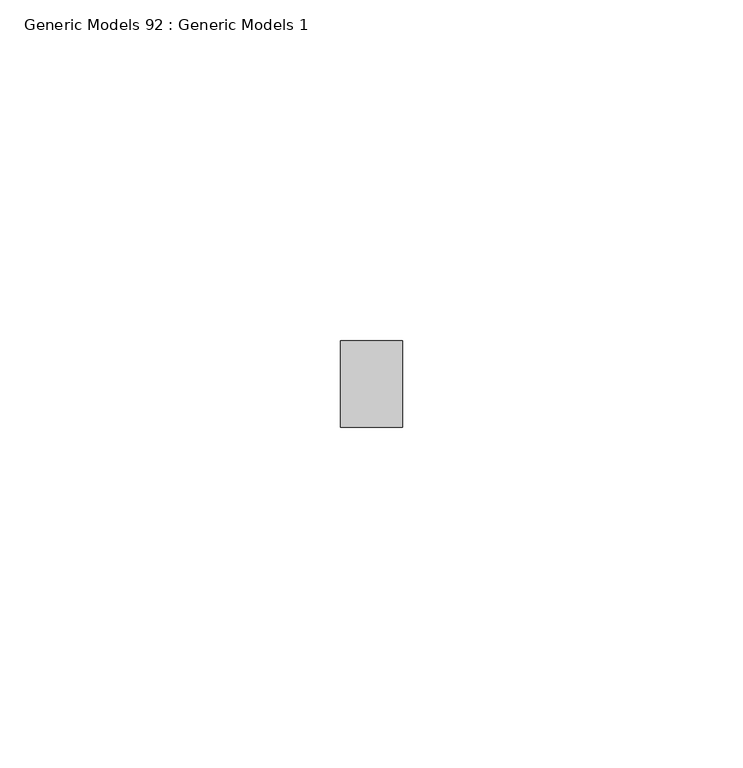
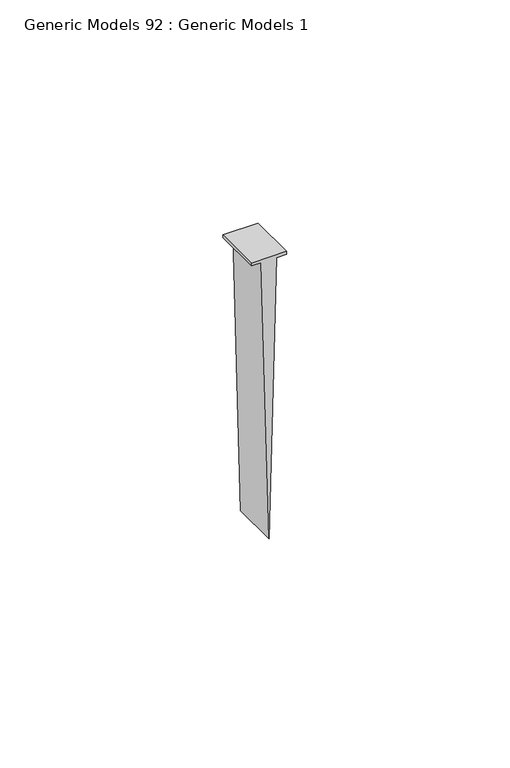
"""IFC4 building model written with IfcOpenShell, lengths in millimetres: proxy geometry, Generic Models 92 : Generic Models 1."""

from ifc_helpers import new_model, si_unit, frame, origin, place, context, project, spatial, polyline, outline, extrude, source, transform, mapped, element, save


def generic_models_92_generic_models_1_05829357(model_context):
    return source(origin(), model_context, "Body", "SweptSolid", [
        extrude(outline(polyline([(67.537912, 48511.0409), (66.744162, 48511.0409), (66.744162, 48513.5907636), (-9.455838, 48515.5875), (66.744162, 48517.5842364), (66.744162, 48520.1341), (67.537912, 48520.1341), (67.537912, 48511.0409)])), frame((0.0, 565.15, 0.0), z_axis=(0.0, 1.0, 0.0), x_axis=(0.0, 0.0, 1.0)), (0.0, 0.0, 1.0), 12.7),
    ])


if __name__ == "__main__":
    model = new_model("IFC4")
    model_context = context("Model", 3, world=origin())
    ifc_project = project(units=[si_unit("LENGTHUNIT", "METRE", prefix="MILLI")], contexts=[model_context])
    site = spatial("IfcSite", under=ifc_project)
    building = spatial("IfcBuilding", under=site)
    placement = place(None, origin())
    generic_models_92_generic_models_1_shape = generic_models_92_generic_models_1_05829357(model_context)
    element("IfcBuildingElementProxy", 1, Name="Generic Models 92 : Generic Models 1", ObjectType="Generic Models 92 : Generic Models 1", at=placement, inside=building, context=model_context, shape_type="MappedRepresentation", body=[
        mapped(generic_models_92_generic_models_1_shape, transform((0.0, 0.0, 0.0), x_axis=(1.0, 0.0, 0.0), y_axis=(0.0, 1.0, 0.0), z_axis=(0.0, 0.0, 1.0))),
    ])
    save(model, "model.ifc")

# Revit data of these elements
# Element 1 (IfcBuildingElementProxy, "Generic Models 92 : Generic Models 1")
#   Materials on its faces: "ATTACH GYPSUM BOARD TO STUDS AND NOT TO TOP TRACK"
# Materials
#   "ATTACH GYPSUM BOARD TO STUDS AND NOT TO TOP TRACK": class "Generic", colour RGB 48 48 48, transparency 0, Cost = 0
